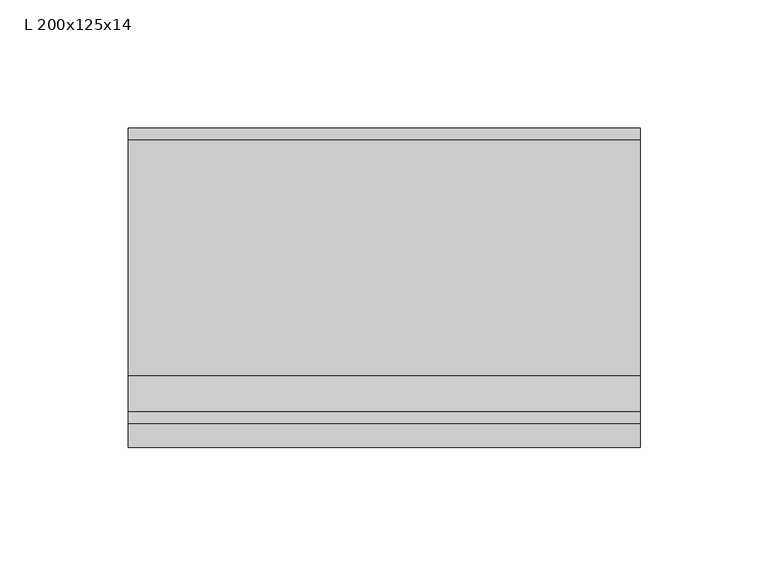
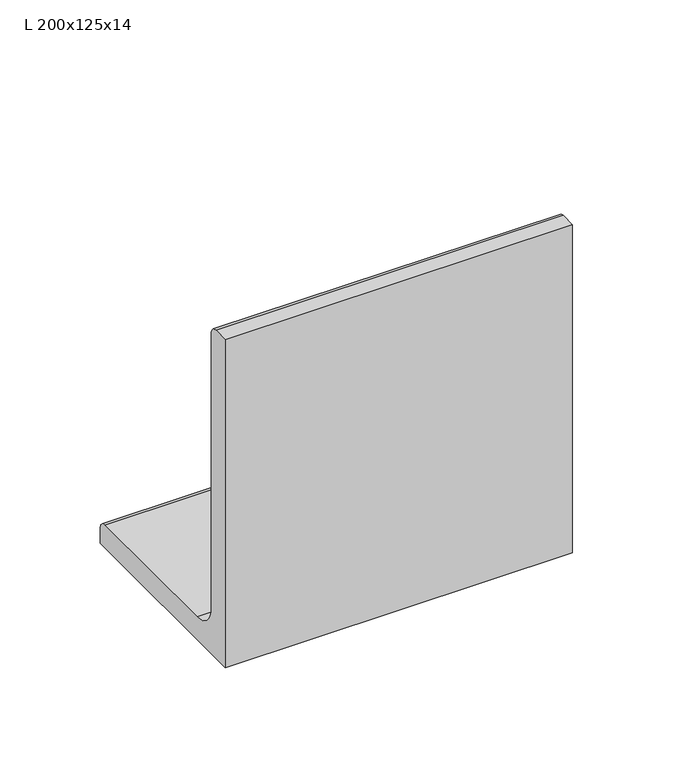
"""IFC4 building model written with IfcOpenShell, lengths in millimetres: beam geometry, Уголок (ГОСТ 8510-86) Балки : L 200x125x14."""

from ifc_helpers import new_model, si_unit, point, frame, frame_2d, origin, place, context, project, spatial, polyline, circle_curve, trimmed, segment, composite_curve, outline, extrude, source, transform, mapped, element, save


def l_200x125x14_cae2d803(model_context):
    return source(origin(), model_context, "Body", "SweptSolid", [
        extrude(outline(composite_curve([segment(polyline([(-29.1, -66.2), (-29.1, 133.8), (-19.8, 133.8)]), True, "CONTINUOUS"), segment(trimmed(circle_curve(frame_2d((-19.8, 129.1)), 4.7), [point((-19.8, 133.8))], [point((-15.1, 129.1))], False, "CARTESIAN"), True, "CONTINUOUS"), segment(polyline([(-15.1, 129.1), (-15.1, -38.2)]), True, "CONTINUOUS"), segment(trimmed(circle_curve(frame_2d((-1.1, -38.2)), 14.0), [point((-15.1, -38.2))], [point((-1.1, -52.2))], True, "CARTESIAN"), True, "CONTINUOUS"), segment(polyline([(-1.1, -52.2), (91.2, -52.2)]), True, "CONTINUOUS"), segment(trimmed(circle_curve(frame_2d((91.2, -56.9)), 4.7), [point((91.2, -52.2))], [point((95.9, -56.9))], False, "CARTESIAN"), True, "CONTINUOUS"), segment(polyline([(95.9, -56.9), (95.9, -66.2), (-29.1, -66.2)]), True, "CONTINUOUS")], self_intersect=False)), frame((-100.0, 0.0, 0.0), z_axis=(1.0, 0.0, 0.0), x_axis=(0.0, 1.0, 0.0)), (0.0, 0.0, 1.0), 200.0),
    ])


if __name__ == "__main__":
    model = new_model("IFC4")
    model_context = context("Model", 3, world=origin())
    ifc_project = project(units=[si_unit("LENGTHUNIT", "METRE", prefix="MILLI")], contexts=[model_context])
    site = spatial("IfcSite", under=ifc_project)
    building = spatial("IfcBuilding", under=site)
    placement = place(None, origin())
    l_200x125x14_shape = l_200x125x14_cae2d803(model_context)
    element("IfcBeam", 1, ObjectType="Уголок (ГОСТ 8510-86) Балки : L 200x125x14", at=placement, inside=building, context=model_context, shape_type="MappedRepresentation", body=[
        mapped(l_200x125x14_shape, transform((0.0, 0.0, 0.0), x_axis=(1.0, 0.0, 0.0), y_axis=(0.0, 1.0, 0.0), z_axis=(0.0, 0.0, 1.0))),
    ])
    save(model, "model.ifc")

# Revit data of these elements
# Type "Уголок (ГОСТ 8510-86) Балки : L 200x125x14"
#   ri = 4.7 mm
#   ra = 14 mm
#   W = 0.337643
#   Vz = 133.8 mm
#   Vy = 95.9 mm
#   Vpz = 66.2 mm
#   Vpy = 29.1 mm
#   Length [instance default] = 1500 mm
#   bf = 125 mm
#   d = 200 mm
#   tf = 14 mm
#   tw = 14 mm
#   A = 0.004387 m²
#   Structural Material [instance default] = Металл - Сталь - 345 МПa
#   Assembly Code = ""
# Element 1 (IfcBeam, "Уголок (ГОСТ 8510-86) Балки : L 200x125x14")
#   Structural Material = C235
#   Materials on its faces: "C235"
# Materials
#   "Металл - Сталь - 345 МПa": class "Металл", colour RGB 247 247 247, transparency 0
#   "C235": class "Не назначено", colour RGB 0 0 0, transparency 0
